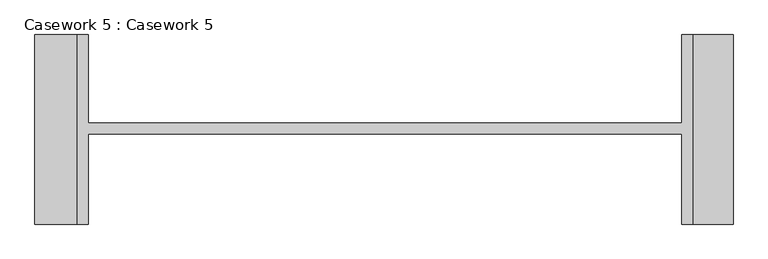
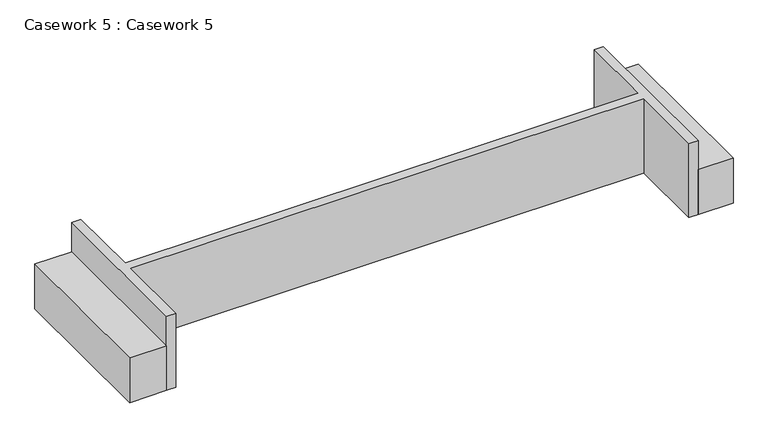
"""IFC4 building model written with IfcOpenShell, lengths in millimetres: furniture geometry, Casework 5 : Casework 5."""

from ifc_helpers import new_model, si_unit, origin, origin_with_axes, place, context, project, spatial, polyline, outline, extrude, source, transform, mapped, element, save


def casework_5_casework_5_e37dcf5b(model_context):
    return source(origin(), model_context, "Body", "SweptSolid", [
        extrude(outline(polyline([(-45711.923082, 271640.9135341), (-45711.923082, 269099.8622246), (-46255.3301106, 269099.8622246), (-46255.3301106, 271640.9135341), (-45711.923082, 271640.9135341)])), origin_with_axes(), (0.0, 0.0, 1.0), 736.6),
        extrude(outline(polyline([(-54498.404085, 271640.9135341), (-54498.404085, 269099.8622246), (-55069.0832901, 269099.8622246), (-55069.0832901, 271640.9135341), (-54498.404085, 271640.9135341)])), origin_with_axes(), (0.0, 0.0, 1.0), 736.6),
        extrude(outline(polyline([(-54355.5266335, 271640.9135341), (-54355.5266335, 270453.7050198), (-46397.0475446, 270453.7050198), (-46397.0475446, 271640.9135341), (-46255.3301106, 271640.9135341), (-46255.3301106, 269099.8622246), (-46397.0475446, 269099.8622246), (-46397.0475446, 270311.8417013), (-54355.5266335, 270311.8417013), (-54355.5266335, 269099.8622246), (-54498.404085, 269099.8622246), (-54498.404085, 271640.9135341), (-54355.5266335, 271640.9135341)])), origin_with_axes(), (0.0, 0.0, 1.0), 1219.2),
    ])


if __name__ == "__main__":
    model = new_model("IFC4")
    model_context = context("Model", 3, world=origin())
    ifc_project = project(units=[si_unit("LENGTHUNIT", "METRE", prefix="MILLI")], contexts=[model_context])
    site = spatial("IfcSite", under=ifc_project)
    building = spatial("IfcBuilding", under=site)
    placement = place(None, origin())
    casework_5_casework_5_shape = casework_5_casework_5_e37dcf5b(model_context)
    element("IfcFurniture", 1, ObjectType="Casework 5 : Casework 5", at=placement, inside=building, context=model_context, shape_type="MappedRepresentation", body=[
        mapped(casework_5_casework_5_shape, transform((0.0, 0.0, 0.0), x_axis=(1.0, 0.0, 0.0), y_axis=(0.0, 1.0, 0.0), z_axis=(0.0, 0.0, 1.0))),
    ])
    save(model, "model.ifc")

# Revit data of these elements
# Element 1 (IfcFurniture, "Casework 5 : Casework 5")
#   Materials on its faces: "1.50\" ASPHALT SURFACE COURSE (E-0.3)"
# Materials
#   "1.50\" ASPHALT SURFACE COURSE (E-0.3)": class "Miscellaneous", colour RGB 164 164 164, transparency 0, Cost = 0
